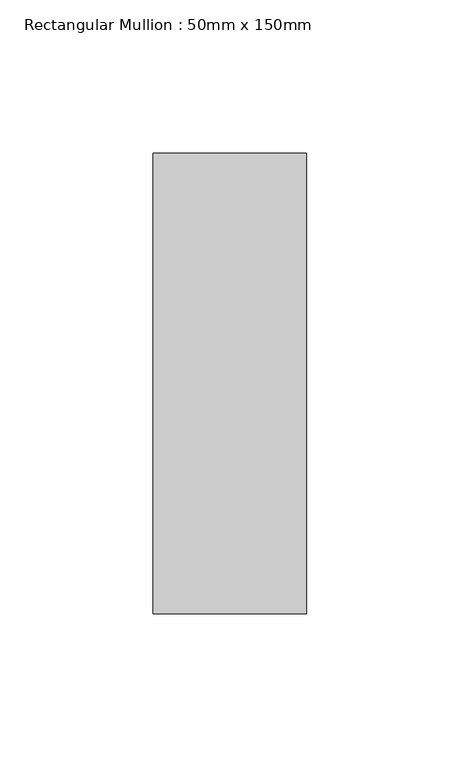
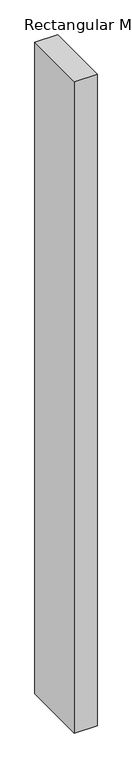
"""IFC4 building model written with IfcOpenShell, lengths in millimetres: member geometry, Rectangular Mullion : 50mm x 150mm."""

from ifc_helpers import new_model, si_unit, frame, origin, place, context, project, spatial, polyline, outline, extrude, source, transform, mapped, element, save


def rectangular_mullion_50mm_x_150mm_7c934e26(model_context):
    return source(origin(), model_context, "Body", "SweptSolid", [
        extrude(outline(polyline([(0.0, 75.0), (0.0, -75.0), (-50.0, -75.0), (-50.0, 75.0), (0.0, 75.0)])), frame((0.0, 0.0, -1515.0930582), z_axis=(0.0, 0.0, 1.0), x_axis=(1.0, 0.0, 0.0)), (0.0, 0.0, 1.0), 1515.0930582),
    ])


if __name__ == "__main__":
    model = new_model("IFC4")
    model_context = context("Model", 3, world=origin())
    ifc_project = project(units=[si_unit("LENGTHUNIT", "METRE", prefix="MILLI")], contexts=[model_context])
    site = spatial("IfcSite", under=ifc_project)
    building = spatial("IfcBuilding", under=site)
    placement = place(None, origin())
    rectangular_mullion_50mm_x_150mm_shape = rectangular_mullion_50mm_x_150mm_7c934e26(model_context)
    element("IfcMember", 1, ObjectType="Rectangular Mullion : 50mm x 150mm", at=placement, inside=building, context=model_context, shape_type="MappedRepresentation", body=[
        mapped(rectangular_mullion_50mm_x_150mm_shape, transform((0.0, 0.0, 0.0), x_axis=(1.0, 0.0, 0.0), y_axis=(0.0, 1.0, 0.0), z_axis=(0.0, 0.0, 1.0))),
    ])
    save(model, "model.ifc")

# Revit data of these elements
# Type "Rectangular Mullion : 50mm x 150mm"
#   built-in parameter 1007304 = 0.492126 (stored number, unit not read)
#   built-in parameter 1007301 = 0.082021 (stored number, unit not read)
#   built-in parameter 1007300 = 0.082021 (stored number, unit not read)
# Element 1 (IfcMember, "Rectangular Mullion : 50mm x 150mm")
#   Materials on its faces: "Aluminum"
# Materials
#   "Aluminum": class "Metal", colour RGB 244 244 244, transparency 0, Description = "Aluminum 6061", Cost = 0
